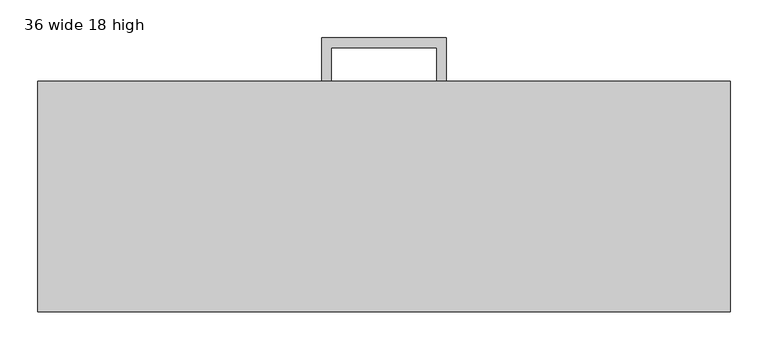
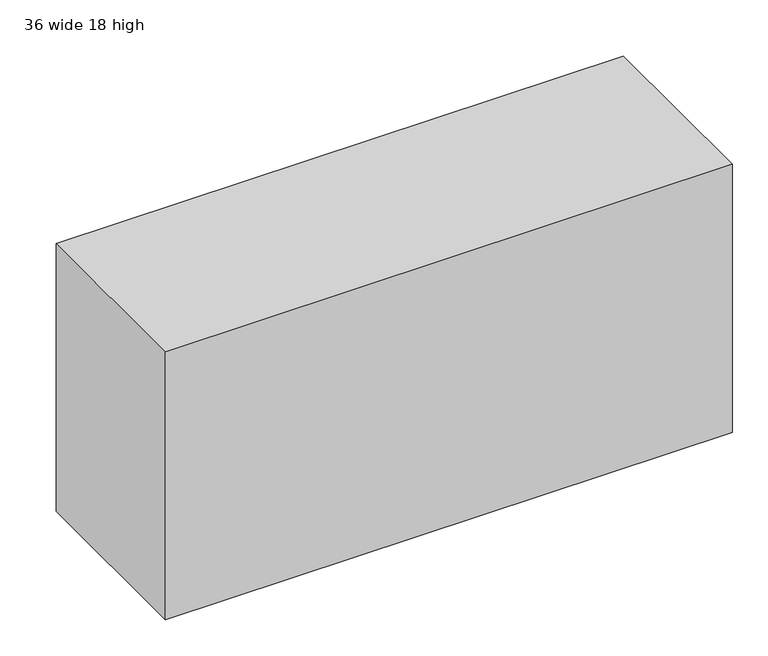
"""IFC4 building model written with IfcOpenShell, lengths in millimetres: furniture geometry, Binder Bin : 36 wide 18 high."""

from ifc_helpers import new_model, si_unit, frame, origin, place, context, project, spatial, polyline, outline, extrude, source, transform, mapped, element, save


def furniture_36_wide_18_high_68bd698f(model_context):
    return source(origin(), model_context, "Body", "SweptSolid", [
        extrude(outline(polyline([(-69.85, 381.0), (-82.55, 381.0), (-82.55, 438.15), (82.55, 438.15), (82.55, 381.0), (69.85, 381.0), (69.85, 425.45), (-69.85, 425.45), (-69.85, 381.0)])), frame((0.0, 0.0, 1568.45), z_axis=(0.0, 0.0, 1.0), x_axis=(1.0, 0.0, 0.0)), (0.0, 0.0, 1.0), 12.7),
        extrude(outline(polyline([(457.2, 76.2), (-457.2, 76.2), (-457.2, 381.0), (457.2, 381.0), (457.2, 76.2)])), frame((0.0, 0.0, 1524.0), z_axis=(0.0, 0.0, 1.0), x_axis=(1.0, 0.0, 0.0)), (0.0, 0.0, 1.0), 457.2),
    ])


if __name__ == "__main__":
    model = new_model("IFC4")
    model_context = context("Model", 3, world=origin())
    ifc_project = project(units=[si_unit("LENGTHUNIT", "METRE", prefix="MILLI")], contexts=[model_context])
    site = spatial("IfcSite", under=ifc_project)
    building = spatial("IfcBuilding", under=site)
    placement = place(None, origin())
    furniture_36_wide_18_high_shape = furniture_36_wide_18_high_68bd698f(model_context)
    element("IfcFurniture", 1, ObjectType="Binder Bin : 36 wide 18 high", at=placement, inside=building, context=model_context, shape_type="MappedRepresentation", body=[
        mapped(furniture_36_wide_18_high_shape, transform((0.0, 0.0, 0.0), x_axis=(1.0, 0.0, 0.0), y_axis=(0.0, 1.0, 0.0), z_axis=(0.0, 0.0, 1.0))),
    ])
    save(model, "model.ifc")

# Revit data of these elements
# Type "Binder Bin : 36 wide 18 high"
#   Model = "BIN-3618"
#   Manufacturer = "Corporate Concepts"
#   Type Mark = "BN-1"
#   Model = "BIN-3618"
#   Manufacturer = "Corporate Concepts"
#   Cost = 625
#   Width = 3' - 0"
#   Mounting Height [instance default] = 4' - 6"
#   Height = 1' - 6"
#   Cost = 625
#   Type Image = Binder Bin.png
#   Default Elevation = 0
# Element 1 (IfcFurniture, "Binder Bin : 36 wide 18 high")
#   Mounting Height = 5' - 0"
